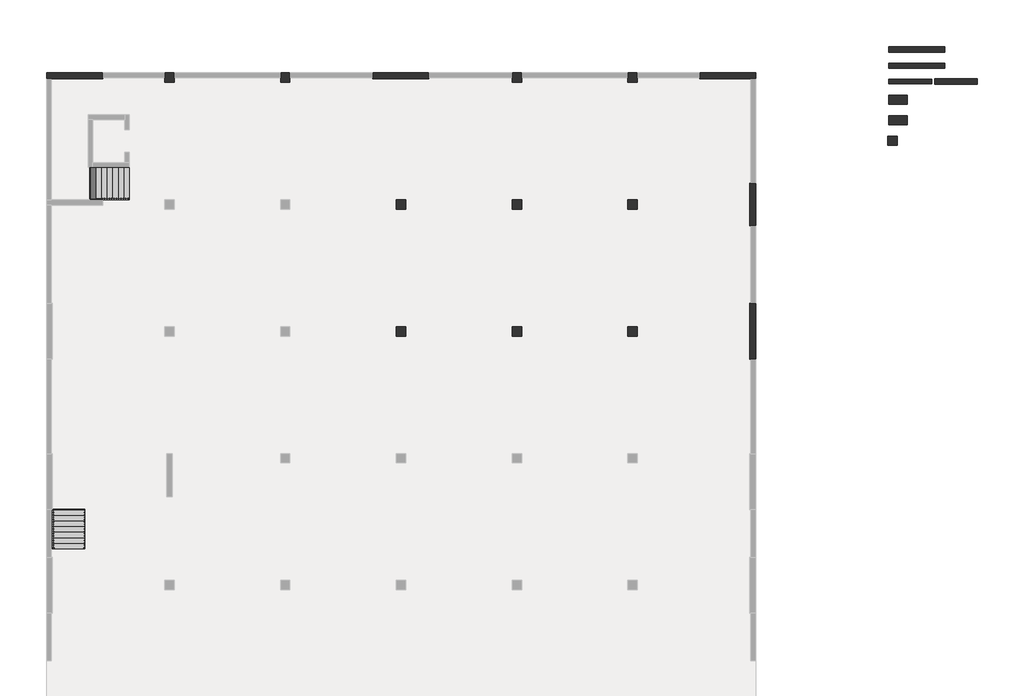
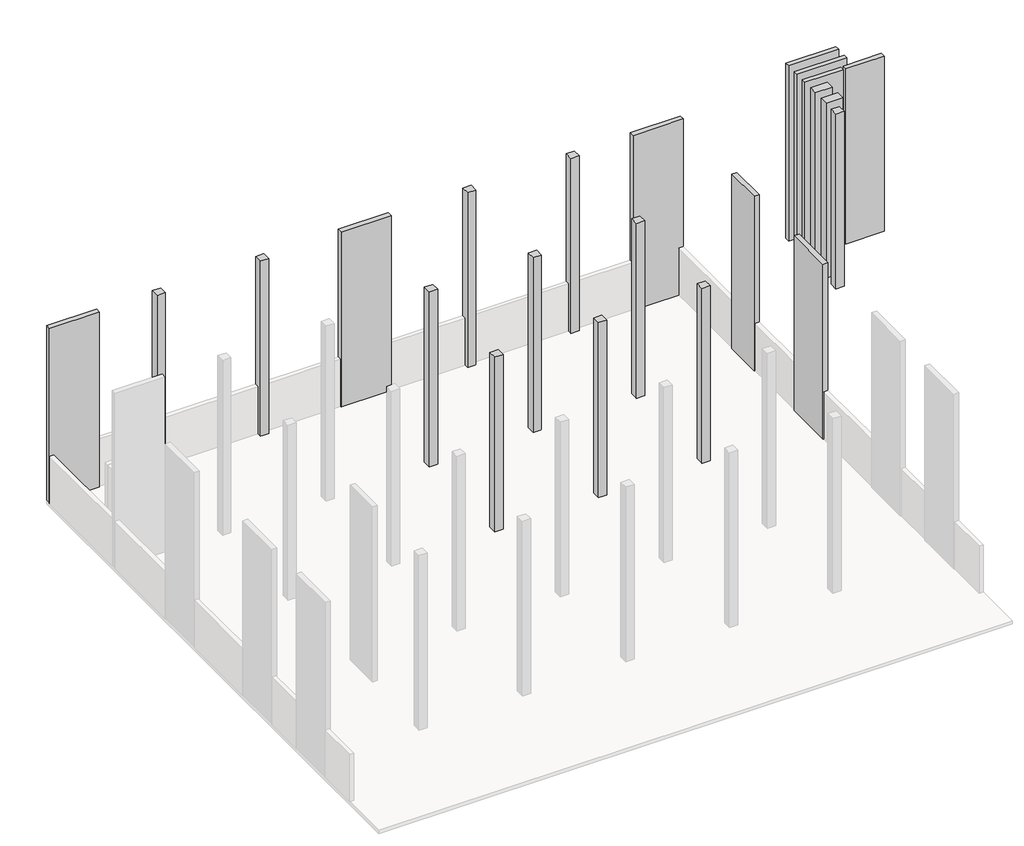
# One storey, part 2 of 2: 22 columns, 3 railings, 2 members, 2 stair flights.
"""IFC4 building model written with IfcOpenShell, lengths in millimetres."""

import ifcopenshell
import ifcopenshell.guid

model = None  # the IFC model being written
_history = None  # IfcOwnerHistory: only IFC2X3 demands one
_inside = {}  # id of a spatial element -> (the spatial element, [elements in it])
_under = {}  # id of a project, library or spatial element -> (it, [spatial elements below it])
_declared = {}  # id of a project -> (the project, [libraries it declares])
_typed = {}  # id of a type object -> (the type object, [elements of that type])
_made_of = {}  # id of a material, layer set ... -> (it, [elements and type objects made of it])


def new_model(schema):
    """Start an empty IFC model of exactly this schema.

    Asked for "IFC4X3", IfcOpenShell would pick the latest addendum, in which some entities
    have other attributes; the version numbers below select the first issue.
    IFC2X3 requires an IfcOwnerHistory on every rooted entity: one is made here for all.
    """
    global model, _history
    if schema == "IFC4X3":
        model = ifcopenshell.file(schema_version=(4, 3, 0, 0))
    else:
        model = ifcopenshell.file(schema=schema)
    _inside.clear()
    _under.clear()
    _declared.clear()
    _typed.clear()
    _made_of.clear()
    _history = None
    if model.schema == "IFC2X3":
        org = make("IfcOrganization", Name="unknown")
        user = make(
            "IfcPersonAndOrganization",
            ThePerson=make("IfcPerson", FamilyName="unknown"),
            TheOrganization=org,
        )
        app = make(
            "IfcApplication",
            ApplicationDeveloper=org,
            Version="unknown",
            ApplicationFullName="unknown",
            ApplicationIdentifier="unknown",
        )
        _history = make(
            "IfcOwnerHistory",
            OwningUser=user,
            OwningApplication=app,
            ChangeAction="ADDED",
            CreationDate=0,
        )
    return model


def make(cls, **values):
    """One entity of the class cls with the attributes given. An attribute that is None is left unset."""
    return model.create_entity(
        cls, **{name: value for name, value in values.items() if value is not None}
    )


def rooted(cls, **values):
    """An entity with a GlobalId (a new one), such as an element, a storey or a relation."""
    return make(cls, GlobalId=ifcopenshell.guid.new(), OwnerHistory=_history, **values)


def si_unit(unit_type, name, prefix=None):
    """IfcSIUnit, for example si_unit("LENGTHUNIT", "METRE", prefix="MILLI")."""
    return make("IfcSIUnit", UnitType=unit_type, Prefix=prefix, Name=name)


def assignment(units):
    """IfcUnitAssignment: the units of a project."""
    return None if units is None else make("IfcUnitAssignment", Units=units)


def point(xyz):
    """IfcCartesianPoint."""
    return None if xyz is None else make("IfcCartesianPoint", Coordinates=xyz)


def direction(xyz):
    """IfcDirection."""
    return None if xyz is None else make("IfcDirection", DirectionRatios=xyz)


def frame(location, z_axis=None, x_axis=None):
    """IfcAxis2Placement3D, a coordinate frame: its origin and axes. An axis left out is left unset."""
    return make(
        "IfcAxis2Placement3D",
        Location=point(location),
        Axis=direction(z_axis),
        RefDirection=direction(x_axis),
    )


def origin():
    """The frame at (0, 0, 0) with its axes left unset."""
    return frame((0.0, 0.0, 0.0))


def place(relative_to, where):
    """IfcLocalPlacement: puts the frame where relative to a parent placement (None: the world)."""
    return make(
        "IfcLocalPlacement", PlacementRelTo=relative_to, RelativePlacement=where
    )


def context(
    kind, dimensions, precision=None, world=None, true_north=None, identifier=None
):
    """IfcGeometricRepresentationContext, for example the 3D "Model" context."""
    return make(
        "IfcGeometricRepresentationContext",
        ContextIdentifier=identifier,
        ContextType=kind,
        CoordinateSpaceDimension=dimensions,
        Precision=precision,
        WorldCoordinateSystem=world,
        TrueNorth=true_north,
    )


def project(units=None, contexts=None):
    """IfcProject with its units and contexts."""
    return rooted(
        "IfcProject",
        Name="project",
        RepresentationContexts=contexts,
        UnitsInContext=assignment(units),
    )


def spatial(cls, under=None, at=None, **own):
    """A site, building, storey or space (cls), placed at a placement, below another one or the project."""
    s = rooted(cls, ObjectPlacement=at, **own)
    if under is not None:
        _under.setdefault(under.id(), (under, []))[1].append(s)
    return s


def polyline(points):
    """IfcPolyline through the points."""
    return make("IfcPolyline", Points=[point(p) for p in points])


def outline(outer, holes=None, kind="AREA"):
    """IfcArbitraryClosedProfileDef: a profile drawn as a closed curve; with holes, ...WithVoids."""
    if holes is None:
        return make("IfcArbitraryClosedProfileDef", ProfileType=kind, OuterCurve=outer)
    return make(
        "IfcArbitraryProfileDefWithVoids",
        ProfileType=kind,
        OuterCurve=outer,
        InnerCurves=holes,
    )


def extrude(swept, where, along, depth):
    """IfcExtrudedAreaSolid: the profile swept, set in the frame where, extruded along a direction by depth."""
    return make(
        "IfcExtrudedAreaSolid",
        SweptArea=swept,
        Position=where,
        ExtrudedDirection=direction(along),
        Depth=depth,
    )


def shape(context_of_items, identifier, shape_type, items):
    """IfcShapeRepresentation: the items that make up one representation, for example the "Body"."""
    return make(
        "IfcShapeRepresentation",
        ContextOfItems=context_of_items,
        RepresentationIdentifier=identifier,
        RepresentationType=shape_type,
        Items=items,
    )


def source(mapping_origin, context_of_items, identifier, shape_type, items):
    """IfcRepresentationMap: a shape defined once, which mapped items show again and again."""
    return make(
        "IfcRepresentationMap",
        MappingOrigin=mapping_origin,
        MappedRepresentation=shape(context_of_items, identifier, shape_type, items),
    )


def transform(
    local_origin,
    x_axis=None,
    y_axis=None,
    z_axis=None,
    scale=None,
    scale2=None,
    scale3=None,
    uniform=True,
):
    """IfcCartesianTransformationOperator3D, or its non-uniform kind. x_axis, y_axis, z_axis: its Axis1, 2, 3."""
    if uniform:
        return make(
            "IfcCartesianTransformationOperator3D",
            Axis1=direction(x_axis),
            Axis2=direction(y_axis),
            LocalOrigin=point(local_origin),
            Scale=scale,
            Axis3=direction(z_axis),
        )
    return make(
        "IfcCartesianTransformationOperator3DnonUniform",
        Axis1=direction(x_axis),
        Axis2=direction(y_axis),
        LocalOrigin=point(local_origin),
        Scale=scale,
        Axis3=direction(z_axis),
        Scale2=scale2,
        Scale3=scale3,
    )


def mapped(mapping_source, mapping_target):
    """IfcMappedItem: shows the shape of a source again, moved by a transform."""
    return make(
        "IfcMappedItem", MappingSource=mapping_source, MappingTarget=mapping_target
    )


def made_of(thing, what):
    """Note that an element or type object is made of a material, layer set ...; save() writes the relation."""
    if what is not None:
        _made_of.setdefault(what.id(), (what, []))[1].append(thing)
    return thing


def element(
    cls,
    number,
    at=None,
    inside=None,
    cuts=None,
    type_object=None,
    material=None,
    context=None,
    identifier="Body",
    shape_type=None,
    held_by="IfcProductDefinitionShape",
    body=None,
    shapes=None,
    **own,
):
    """One element of the class cls, such as IfcWall. Its Tag is "e" and its number.

    at: its placement. inside: the storey or other place that contains it. cuts: it is an
    opening in that element (IfcRelVoidsElement). A single representation is given by context,
    identifier, shape_type and body (its items); several are given by shapes. held_by: the class
    of the entity that holds the representations. save() writes the other relations.
    """
    e = rooted(cls, Tag="e%d" % number, ObjectPlacement=at, **own)
    if body is not None:
        shapes = [shape(context, identifier, shape_type, body)]
    if shapes is not None:
        e.Representation = make(held_by, Representations=shapes)
    if inside is not None:
        _inside.setdefault(inside.id(), (inside, []))[1].append(e)
    if cuts is not None:
        rooted(
            "IfcRelVoidsElement", RelatingBuildingElement=cuts, RelatedOpeningElement=e
        )
    if type_object is not None:
        _typed.setdefault(type_object.id(), (type_object, []))[1].append(e)
    return made_of(e, material)


def aggregate(whole, parts):
    """IfcRelAggregates: a whole, such as a stair, and the parts it consists of."""
    return rooted("IfcRelAggregates", RelatingObject=whole, RelatedObjects=parts)


def save(model, path):
    """Write the relations noted so far, then the file.

    IfcRelAggregates (storeys below a building ...), IfcRelContainedInSpatialStructure (elements
    in a storey), IfcRelDefinesByType, IfcRelAssociatesMaterial and IfcRelDeclares: one each for
    every whole, place, type object, material and project.
    """
    for whole, parts in _under.values():
        aggregate(whole, parts)
    for where, things in _inside.values():
        rooted(
            "IfcRelContainedInSpatialStructure",
            RelatedElements=things,
            RelatingStructure=where,
        )
    for kind, things in _typed.values():
        rooted("IfcRelDefinesByType", RelatedObjects=things, RelatingType=kind)
    for what, things in _made_of.values():
        rooted("IfcRelAssociatesMaterial", RelatedObjects=things, RelatingMaterial=what)
    for by, libraries in _declared.values():
        rooted("IfcRelDeclares", RelatingContext=by, RelatedDefinitions=libraries)
    model.write(path)


def m_rectangular_column_100x50_89a3459c(model_context):
    return source(origin(), model_context, "Body", "SweptSolid", [
        extrude(outline(polyline([(500.0, 250.0), (500.0, -250.0), (-500.0, -250.0), (-500.0, 250.0), (500.0, 250.0)])), frame((0.0, 0.0, -3200.0), z_axis=(0.0, 0.0, 1.0), x_axis=(1.0, 0.0, 0.0)), (0.0, 0.0, 1.0), 11100.0),
    ])


def m_rectangular_column_230x25_da6e8c6c(model_context):
    return source(origin(), model_context, "Body", "SweptSolid", [
        extrude(outline(polyline([(1150.0, 125.0), (1150.0, -125.0), (-1150.0, -125.0), (-1150.0, 125.0), (1150.0, 125.0)])), frame((0.0, 0.0, -3200.0), z_axis=(0.0, 0.0, 1.0), x_axis=(1.0, 0.0, 0.0)), (0.0, 0.0, 1.0), 11100.0),
    ])


def m_rectangular_column_230x30_624f9335(model_context):
    return source(origin(), model_context, "Body", "SweptSolid", [
        extrude(outline(polyline([(1150.0, 150.0), (1150.0, -150.0), (-1150.0, -150.0), (-1150.0, 150.0), (1150.0, 150.0)])), frame((0.0, 0.0, -3200.0), z_axis=(0.0, 0.0, 1.0), x_axis=(1.0, 0.0, 0.0)), (0.0, 0.0, 1.0), 11100.0),
    ])


def m_rectangular_column_300x25_b7e4e278(model_context):
    return source(origin(), model_context, "Body", "SweptSolid", [
        extrude(outline(polyline([(1500.0, 125.0), (1500.0, -125.0), (-1500.0, -125.0), (-1500.0, 125.0), (1500.0, 125.0)])), frame((0.0, 0.0, -3200.0), z_axis=(0.0, 0.0, 1.0), x_axis=(1.0, 0.0, 0.0)), (0.0, 0.0, 1.0), 11100.0),
    ])


def m_rectangular_column_300x30_b7aa0491(model_context):
    return source(origin(), model_context, "Body", "SweptSolid", [
        extrude(outline(polyline([(1500.0, 150.0), (1500.0, -150.0), (-1500.0, -150.0), (-1500.0, 150.0), (1500.0, 150.0)])), frame((0.0, 0.0, -3200.0), z_axis=(0.0, 0.0, 1.0), x_axis=(1.0, 0.0, 0.0)), (0.0, 0.0, 1.0), 11100.0),
    ])


def m_rectangular_column_50x50_3a95f3c9(model_context):
    return source(origin(), model_context, "Body", "SweptSolid", [
        extrude(outline(polyline([(250.0, 250.0), (250.0, -250.0), (-250.0, -250.0), (-250.0, 250.0), (250.0, 250.0)])), frame((0.0, 0.0, -3200.0), z_axis=(0.0, 0.0, 1.0), x_axis=(1.0, 0.0, 0.0)), (0.0, 0.0, 1.0), 11100.0),
    ])


def stair_flight_50mm_tread_13mm_riser_a4aa0c66(model_context):
    return source(origin(), model_context, "Body", "SweptSolid", [
        extrude(outline(polyline([(-13456.918089, 12730.6768963), (-13444.418089, 12730.6768963), (-13444.418089, 11030.6768963), (-13456.918089, 11030.6768963), (-13456.918089, 12730.6768963)])), frame((0.0, 0.0, -3200.0), z_axis=(0.0, 0.0, 1.0), x_axis=(1.0, 0.0, 0.0)), (0.0, 0.0, 1.0), 127.7777778),
        extrude(outline(polyline([(-13744.418089, 11030.6768963), (-13744.418089, 12730.6768963), (-13444.418089, 12730.6768963), (-13444.418089, 11030.6768963), (-13744.418089, 11030.6768963)])), frame((0.0, 0.0, -3072.2222222), z_axis=(0.0, 0.0, 1.0), x_axis=(1.0, 0.0, 0.0)), (0.0, 0.0, 1.0), 50.0),
        extrude(outline(polyline([(-13756.918089, 12730.6768963), (-13744.418089, 12730.6768963), (-13744.418089, 11030.6768963), (-13756.918089, 11030.6768963), (-13756.918089, 12730.6768963)])), frame((0.0, 0.0, -3072.2222222), z_axis=(0.0, 0.0, 1.0), x_axis=(1.0, 0.0, 0.0)), (0.0, 0.0, 1.0), 177.7777778),
        extrude(outline(polyline([(-14044.418089, 11030.6768963), (-14044.418089, 12730.6768963), (-13744.418089, 12730.6768963), (-13744.418089, 11030.6768963), (-14044.418089, 11030.6768963)])), frame((0.0, 0.0, -2894.4444444), z_axis=(0.0, 0.0, 1.0), x_axis=(1.0, 0.0, 0.0)), (0.0, 0.0, 1.0), 50.0),
        extrude(outline(polyline([(-14056.918089, 12730.6768963), (-14044.418089, 12730.6768963), (-14044.418089, 11030.6768963), (-14056.918089, 11030.6768963), (-14056.918089, 12730.6768963)])), frame((0.0, 0.0, -2894.4444444), z_axis=(0.0, 0.0, 1.0), x_axis=(1.0, 0.0, 0.0)), (0.0, 0.0, 1.0), 177.7777778),
        extrude(outline(polyline([(-14344.418089, 11030.6768963), (-14344.418089, 12730.6768963), (-14044.418089, 12730.6768963), (-14044.418089, 11030.6768963), (-14344.418089, 11030.6768963)])), frame((0.0, 0.0, -2716.6666667), z_axis=(0.0, 0.0, 1.0), x_axis=(1.0, 0.0, 0.0)), (0.0, 0.0, 1.0), 50.0),
        extrude(outline(polyline([(-14356.918089, 12730.6768963), (-14344.418089, 12730.6768963), (-14344.418089, 11030.6768963), (-14356.918089, 11030.6768963), (-14356.918089, 12730.6768963)])), frame((0.0, 0.0, -2716.6666667), z_axis=(0.0, 0.0, 1.0), x_axis=(1.0, 0.0, 0.0)), (0.0, 0.0, 1.0), 177.7777778),
        extrude(outline(polyline([(-14644.418089, 11030.6768963), (-14644.418089, 12730.6768963), (-14344.418089, 12730.6768963), (-14344.418089, 11030.6768963), (-14644.418089, 11030.6768963)])), frame((0.0, 0.0, -2538.8888889), z_axis=(0.0, 0.0, 1.0), x_axis=(1.0, 0.0, 0.0)), (0.0, 0.0, 1.0), 50.0),
        extrude(outline(polyline([(-14656.918089, 12730.6768963), (-14644.418089, 12730.6768963), (-14644.418089, 11030.6768963), (-14656.918089, 11030.6768963), (-14656.918089, 12730.6768963)])), frame((0.0, 0.0, -2538.8888889), z_axis=(0.0, 0.0, 1.0), x_axis=(1.0, 0.0, 0.0)), (0.0, 0.0, 1.0), 177.7777778),
        extrude(outline(polyline([(-14944.418089, 11030.6768963), (-14944.418089, 12730.6768963), (-14644.418089, 12730.6768963), (-14644.418089, 11030.6768963), (-14944.418089, 11030.6768963)])), frame((0.0, 0.0, -2361.1111111), z_axis=(0.0, 0.0, 1.0), x_axis=(1.0, 0.0, 0.0)), (0.0, 0.0, 1.0), 50.0),
        extrude(outline(polyline([(-14956.918089, 12730.6768963), (-14944.418089, 12730.6768963), (-14944.418089, 11030.6768963), (-14956.918089, 11030.6768963), (-14956.918089, 12730.6768963)])), frame((0.0, 0.0, -2361.1111111), z_axis=(0.0, 0.0, 1.0), x_axis=(1.0, 0.0, 0.0)), (0.0, 0.0, 1.0), 177.7777778),
        extrude(outline(polyline([(-15244.418089, 11030.6768963), (-15244.418089, 12730.6768963), (-14944.418089, 12730.6768963), (-14944.418089, 11030.6768963), (-15244.418089, 11030.6768963)])), frame((0.0, 0.0, -2183.3333333), z_axis=(0.0, 0.0, 1.0), x_axis=(1.0, 0.0, 0.0)), (0.0, 0.0, 1.0), 50.0),
        extrude(outline(polyline([(-15256.918089, 12730.6768963), (-15244.418089, 12730.6768963), (-15244.418089, 11030.6768963), (-15256.918089, 11030.6768963), (-15256.918089, 12730.6768963)])), frame((0.0, 0.0, -2183.3333333), z_axis=(0.0, 0.0, 1.0), x_axis=(1.0, 0.0, 0.0)), (0.0, 0.0, 1.0), 177.7777778),
        extrude(outline(polyline([(-15556.918089, 12730.6768963), (-15544.418089, 12730.6768963), (-15544.418089, 11030.6768963), (-15556.918089, 11030.6768963), (-15556.918089, 12730.6768963)])), frame((0.0, 0.0, -2005.5555556), z_axis=(0.0, 0.0, 1.0), x_axis=(1.0, 0.0, 0.0)), (0.0, 0.0, 1.0), 177.7777778),
        extrude(outline(polyline([(-15544.418089, 11030.6768963), (-15544.418089, 12730.6768963), (-15244.418089, 12730.6768963), (-15244.418089, 11030.6768963), (-15544.418089, 11030.6768963)])), frame((0.0, 0.0, -2005.5555556), z_axis=(0.0, 0.0, 1.0), x_axis=(1.0, 0.0, 0.0)), (0.0, 0.0, 1.0), 50.0),
    ])


def stair_flight_50mm_tread_13mm_riser_6111fc84(model_context):
    return source(origin(), model_context, "Body", "SweptSolid", [
        extrude(outline(polyline([(-15825.2814495, -7705.5731037), (-15825.2814495, -7718.0731037), (-17525.2814495, -7718.0731037), (-17525.2814495, -7705.5731037), (-15825.2814495, -7705.5731037)])), frame((0.0, 0.0, -3200.0), z_axis=(0.0, 0.0, 1.0), x_axis=(1.0, 0.0, 0.0)), (0.0, 0.0, 1.0), 83.3333333),
        extrude(outline(polyline([(-17525.2814495, -7418.0731037), (-15825.2814495, -7418.0731037), (-15825.2814495, -7718.0731037), (-17525.2814495, -7718.0731037), (-17525.2814495, -7418.0731037)])), frame((0.0, 0.0, -3116.6666667), z_axis=(0.0, 0.0, 1.0), x_axis=(1.0, 0.0, 0.0)), (0.0, 0.0, 1.0), 50.0),
        extrude(outline(polyline([(-15825.2814495, -7405.5731037), (-15825.2814495, -7418.0731037), (-17525.2814495, -7418.0731037), (-17525.2814495, -7405.5731037), (-15825.2814495, -7405.5731037)])), frame((0.0, 0.0, -3116.6666667), z_axis=(0.0, 0.0, 1.0), x_axis=(1.0, 0.0, 0.0)), (0.0, 0.0, 1.0), 133.3333333),
        extrude(outline(polyline([(-17525.2814495, -7118.0731037), (-15825.2814495, -7118.0731037), (-15825.2814495, -7418.0731037), (-17525.2814495, -7418.0731037), (-17525.2814495, -7118.0731037)])), frame((0.0, 0.0, -2983.3333333), z_axis=(0.0, 0.0, 1.0), x_axis=(1.0, 0.0, 0.0)), (0.0, 0.0, 1.0), 50.0),
        extrude(outline(polyline([(-15825.2814495, -7105.5731037), (-15825.2814495, -7118.0731037), (-17525.2814495, -7118.0731037), (-17525.2814495, -7105.5731037), (-15825.2814495, -7105.5731037)])), frame((0.0, 0.0, -2983.3333333), z_axis=(0.0, 0.0, 1.0), x_axis=(1.0, 0.0, 0.0)), (0.0, 0.0, 1.0), 133.3333333),
        extrude(outline(polyline([(-17525.2814495, -6818.0731037), (-15825.2814495, -6818.0731037), (-15825.2814495, -7118.0731037), (-17525.2814495, -7118.0731037), (-17525.2814495, -6818.0731037)])), frame((0.0, 0.0, -2850.0), z_axis=(0.0, 0.0, 1.0), x_axis=(1.0, 0.0, 0.0)), (0.0, 0.0, 1.0), 50.0),
        extrude(outline(polyline([(-15825.2814495, -6805.5731037), (-15825.2814495, -6818.0731037), (-17525.2814495, -6818.0731037), (-17525.2814495, -6805.5731037), (-15825.2814495, -6805.5731037)])), frame((0.0, 0.0, -2850.0), z_axis=(0.0, 0.0, 1.0), x_axis=(1.0, 0.0, 0.0)), (0.0, 0.0, 1.0), 133.3333333),
        extrude(outline(polyline([(-17525.2814495, -6518.0731037), (-15825.2814495, -6518.0731037), (-15825.2814495, -6818.0731037), (-17525.2814495, -6818.0731037), (-17525.2814495, -6518.0731037)])), frame((0.0, 0.0, -2716.6666667), z_axis=(0.0, 0.0, 1.0), x_axis=(1.0, 0.0, 0.0)), (0.0, 0.0, 1.0), 50.0),
        extrude(outline(polyline([(-15825.2814495, -6505.5731037), (-15825.2814495, -6518.0731037), (-17525.2814495, -6518.0731037), (-17525.2814495, -6505.5731037), (-15825.2814495, -6505.5731037)])), frame((0.0, 0.0, -2716.6666667), z_axis=(0.0, 0.0, 1.0), x_axis=(1.0, 0.0, 0.0)), (0.0, 0.0, 1.0), 133.3333333),
        extrude(outline(polyline([(-17525.2814495, -6218.0731037), (-15825.2814495, -6218.0731037), (-15825.2814495, -6518.0731037), (-17525.2814495, -6518.0731037), (-17525.2814495, -6218.0731037)])), frame((0.0, 0.0, -2583.3333333), z_axis=(0.0, 0.0, 1.0), x_axis=(1.0, 0.0, 0.0)), (0.0, 0.0, 1.0), 50.0),
        extrude(outline(polyline([(-15825.2814495, -6205.5731037), (-15825.2814495, -6218.0731037), (-17525.2814495, -6218.0731037), (-17525.2814495, -6205.5731037), (-15825.2814495, -6205.5731037)])), frame((0.0, 0.0, -2583.3333333), z_axis=(0.0, 0.0, 1.0), x_axis=(1.0, 0.0, 0.0)), (0.0, 0.0, 1.0), 133.3333333),
        extrude(outline(polyline([(-17525.2814495, -5918.0731037), (-15825.2814495, -5918.0731037), (-15825.2814495, -6218.0731037), (-17525.2814495, -6218.0731037), (-17525.2814495, -5918.0731037)])), frame((0.0, 0.0, -2450.0), z_axis=(0.0, 0.0, 1.0), x_axis=(1.0, 0.0, 0.0)), (0.0, 0.0, 1.0), 50.0),
        extrude(outline(polyline([(-15825.2814495, -5905.5731037), (-15825.2814495, -5918.0731037), (-17525.2814495, -5918.0731037), (-17525.2814495, -5905.5731037), (-15825.2814495, -5905.5731037)])), frame((0.0, 0.0, -2450.0), z_axis=(0.0, 0.0, 1.0), x_axis=(1.0, 0.0, 0.0)), (0.0, 0.0, 1.0), 133.3333333),
        extrude(outline(polyline([(-15825.2814495, -5605.5731037), (-15825.2814495, -5618.0731037), (-17525.2814495, -5618.0731037), (-17525.2814495, -5605.5731037), (-15825.2814495, -5605.5731037)])), frame((0.0, 0.0, -2316.6666667), z_axis=(0.0, 0.0, 1.0), x_axis=(1.0, 0.0, 0.0)), (0.0, 0.0, 1.0), 133.3333333),
        extrude(outline(polyline([(-17525.2814495, -5618.0731037), (-15825.2814495, -5618.0731037), (-15825.2814495, -5918.0731037), (-17525.2814495, -5918.0731037), (-17525.2814495, -5618.0731037)])), frame((0.0, 0.0, -2316.6666667), z_axis=(0.0, 0.0, 1.0), x_axis=(1.0, 0.0, 0.0)), (0.0, 0.0, 1.0), 50.0),
    ])


model = new_model("IFC4")

# Units and contexts
model_context = context("Model", 3, world=origin())
ifc_project = project(units=[si_unit("LENGTHUNIT", "METRE", prefix="MILLI")], contexts=[model_context])

# Site, building, storey
site = spatial("IfcSite", under=ifc_project)
building = spatial("IfcBuilding", under=site)
storey = spatial("IfcBuildingStorey", under=building, Name="Bodrumi", Elevation=-3200.0)

# Columns
placement = place(None, origin())
m_rectangular_column_100x50_shape = m_rectangular_column_100x50_89a3459c(model_context)
element("IfcColumn", 1, ObjectType="M_Rectangular Column : 100x50", at=placement, inside=storey, context=model_context, shape_type="MappedRepresentation", body=[
    mapped(m_rectangular_column_100x50_shape, transform((27767.4045961, 16346.6713325, 0.0), x_axis=(1.0, 0.0, 0.0), y_axis=(0.0, 1.0, 0.0), z_axis=(0.0, 0.0, 1.0))),
])
element("IfcColumn", 2, ObjectType="M_Rectangular Column : 100x50", at=placement, inside=storey, context=model_context, shape_type="MappedRepresentation", body=[
    mapped(m_rectangular_column_100x50_shape, transform((27767.4045961, 15246.6713325, 0.0), x_axis=(1.0, 0.0, 0.0), y_axis=(0.0, 1.0, 0.0), z_axis=(0.0, 0.0, 1.0))),
])
m_rectangular_column_230x25_shape = m_rectangular_column_230x25_da6e8c6c(model_context)
element("IfcColumn", 3, ObjectType="M_Rectangular Column : 230x25", at=placement, inside=storey, context=model_context, shape_type="MappedRepresentation", body=[
    mapped(m_rectangular_column_230x25_shape, transform((28417.4045961, 17321.6713325, 0.0), x_axis=(1.0, 0.0, 0.0), y_axis=(0.0, 1.0, 0.0), z_axis=(0.0, 0.0, 1.0))),
])
m_rectangular_column_230x30_shape = m_rectangular_column_230x30_624f9335(model_context)
element("IfcColumn", 4, ObjectType="M_Rectangular Column : 230x30", at=placement, inside=storey, context=model_context, shape_type="MappedRepresentation", body=[
    mapped(m_rectangular_column_230x30_shape, transform((30867.9046685, 17321.6713325, 0.0), x_axis=(1.0, 0.0, 0.0), y_axis=(0.0, 1.0, 0.0), z_axis=(0.0, 0.0, 1.0))),
])
element("IfcColumn", 5, ObjectType="M_Rectangular Column : 230x30", at=placement, inside=storey, context=model_context, shape_type="MappedRepresentation", body=[
    mapped(m_rectangular_column_230x30_shape, transform((19975.581911, 10730.6768963, 0.0), x_axis=(0.0, 1.0, 0.0), y_axis=(-1.0, 0.0, 0.0), z_axis=(0.0, 0.0, 1.0))),
])
m_rectangular_column_300x25_shape = m_rectangular_column_300x25_b7e4e278(model_context)
element("IfcColumn", 6, ObjectType="M_Rectangular Column : 300x25", at=placement, inside=storey, context=model_context, shape_type="MappedRepresentation", body=[
    mapped(m_rectangular_column_300x25_shape, transform((28767.4045961, 18171.6713325, 0.0), x_axis=(1.0, 0.0, 0.0), y_axis=(0.0, 1.0, 0.0), z_axis=(0.0, 0.0, 1.0))),
])
element("IfcColumn", 7, ObjectType="M_Rectangular Column : 300x30", at=placement, inside=storey, context=model_context, shape_type="SweptSolid", body=[
    extrude(outline(polyline([(-14874.418089, 17780.6768963), (-14874.418089, 17480.6768963), (-17874.418089, 17480.6768963), (-17874.418089, 17780.6768963), (-14874.418089, 17780.6768963)])), frame((0.0, 0.0, -3200.0), z_axis=(0.0, 0.0, 1.0), x_axis=(1.0, 0.0, 0.0)), (0.0, 0.0, 1.0), 11100.0),
])
m_rectangular_column_300x30_shape = m_rectangular_column_300x30_b7aa0491(model_context)
element("IfcColumn", 8, ObjectType="M_Rectangular Column : 300x30", at=placement, inside=storey, context=model_context, shape_type="MappedRepresentation", body=[
    mapped(m_rectangular_column_300x30_shape, transform((28767.4045961, 19046.6713325, 0.0), x_axis=(1.0, 0.0, 0.0), y_axis=(0.0, 1.0, 0.0), z_axis=(0.0, 0.0, 1.0))),
])
element("IfcColumn", 9, ObjectType="M_Rectangular Column : 300x30", at=placement, inside=storey, context=model_context, shape_type="MappedRepresentation", body=[
    mapped(m_rectangular_column_300x30_shape, transform((18625.581911, 17630.6768963, 0.0), x_axis=(1.0, 0.0, 0.0), y_axis=(0.0, 1.0, 0.0), z_axis=(0.0, 0.0, 1.0))),
])
element("IfcColumn", 10, ObjectType="M_Rectangular Column : 300x30", at=placement, inside=storey, context=model_context, shape_type="MappedRepresentation", body=[
    mapped(m_rectangular_column_300x30_shape, transform((1115.581911, 17630.6768963, 0.0), x_axis=(1.0, 0.0, 0.0), y_axis=(0.0, 1.0, 0.0), z_axis=(0.0, 0.0, 1.0))),
])
element("IfcColumn", 11, ObjectType="M_Rectangular Column : 300x30", at=placement, inside=storey, context=model_context, shape_type="MappedRepresentation", body=[
    mapped(m_rectangular_column_300x30_shape, transform((19975.581911, 3930.6768963, 0.0), x_axis=(0.0, 1.0, 0.0), y_axis=(-1.0, 0.0, 0.0), z_axis=(0.0, 0.0, 1.0))),
])
m_rectangular_column_50x50_shape = m_rectangular_column_50x50_3a95f3c9(model_context)
element("IfcColumn", 12, ObjectType="M_Rectangular Column : 50x50", at=placement, inside=storey, context=model_context, shape_type="MappedRepresentation", body=[
    mapped(m_rectangular_column_50x50_shape, transform((27471.1352536, 14146.6713325, 0.0), x_axis=(1.0, 0.0, 0.0), y_axis=(0.0, 1.0, 0.0), z_axis=(0.0, 0.0, 1.0))),
])
element("IfcColumn", 13, ObjectType="M_Rectangular Column : 50x50", at=placement, inside=storey, context=model_context, shape_type="MappedRepresentation", body=[
    mapped(m_rectangular_column_50x50_shape, transform((13535.581911, 3930.6768963, 0.0), x_axis=(1.0, 0.0, 0.0), y_axis=(0.0, 1.0, 0.0), z_axis=(0.0, 0.0, 1.0))),
])
element("IfcColumn", 14, ObjectType="M_Rectangular Column : 50x50", at=placement, inside=storey, context=model_context, shape_type="MappedRepresentation", body=[
    mapped(m_rectangular_column_50x50_shape, transform((13535.581911, 17530.6768963, 0.0), x_axis=(1.0, 0.0, 0.0), y_axis=(0.0, 1.0, 0.0), z_axis=(0.0, 0.0, 1.0))),
])
element("IfcColumn", 15, ObjectType="M_Rectangular Column : 50x50", at=placement, inside=storey, context=model_context, shape_type="MappedRepresentation", body=[
    mapped(m_rectangular_column_50x50_shape, transform((7335.581911, 17530.6768963, 0.0), x_axis=(1.0, 0.0, 0.0), y_axis=(0.0, 1.0, 0.0), z_axis=(0.0, 0.0, 1.0))),
])
element("IfcColumn", 16, ObjectType="M_Rectangular Column : 50x50", at=placement, inside=storey, context=model_context, shape_type="MappedRepresentation", body=[
    mapped(m_rectangular_column_50x50_shape, transform((-5084.418089, 17530.6768963, 0.0), x_axis=(1.0, 0.0, 0.0), y_axis=(0.0, 1.0, 0.0), z_axis=(0.0, 0.0, 1.0))),
])
element("IfcColumn", 17, ObjectType="M_Rectangular Column : 50x50", at=placement, inside=storey, context=model_context, shape_type="MappedRepresentation", body=[
    mapped(m_rectangular_column_50x50_shape, transform((-11284.418089, 17530.6768963, 0.0), x_axis=(1.0, 0.0, 0.0), y_axis=(0.0, 1.0, 0.0), z_axis=(0.0, 0.0, 1.0))),
])
element("IfcColumn", 18, ObjectType="M_Rectangular Column : 50x50", at=placement, inside=storey, context=model_context, shape_type="MappedRepresentation", body=[
    mapped(m_rectangular_column_50x50_shape, transform((1115.581911, 10730.6768963, 0.0), x_axis=(1.0, 0.0, 0.0), y_axis=(0.0, 1.0, 0.0), z_axis=(0.0, 0.0, 1.0))),
])
element("IfcColumn", 19, ObjectType="M_Rectangular Column : 50x50", at=placement, inside=storey, context=model_context, shape_type="MappedRepresentation", body=[
    mapped(m_rectangular_column_50x50_shape, transform((7335.581911, 10730.6768963, 0.0), x_axis=(1.0, 0.0, 0.0), y_axis=(0.0, 1.0, 0.0), z_axis=(0.0, 0.0, 1.0))),
])
element("IfcColumn", 20, ObjectType="M_Rectangular Column : 50x50", at=placement, inside=storey, context=model_context, shape_type="MappedRepresentation", body=[
    mapped(m_rectangular_column_50x50_shape, transform((13535.581911, 10730.6768963, 0.0), x_axis=(1.0, 0.0, 0.0), y_axis=(0.0, 1.0, 0.0), z_axis=(0.0, 0.0, 1.0))),
])
element("IfcColumn", 21, ObjectType="M_Rectangular Column : 50x50", at=placement, inside=storey, context=model_context, shape_type="MappedRepresentation", body=[
    mapped(m_rectangular_column_50x50_shape, transform((1115.581911, 3930.6768963, 0.0), x_axis=(1.0, 0.0, 0.0), y_axis=(0.0, 1.0, 0.0), z_axis=(0.0, 0.0, 1.0))),
])
element("IfcColumn", 22, ObjectType="M_Rectangular Column : 50x50", at=placement, inside=storey, context=model_context, shape_type="MappedRepresentation", body=[
    mapped(m_rectangular_column_50x50_shape, transform((7335.581911, 3930.6768963, 0.0), x_axis=(1.0, 0.0, 0.0), y_axis=(0.0, 1.0, 0.0), z_axis=(0.0, 0.0, 1.0))),
])

# Members
element("IfcMember", 23, ObjectType="Stringer - 50mm Width", at=placement, inside=storey, context=model_context, shape_type="SweptSolid", body=[
    extrude(outline(polyline([(-3200.0, -13444.418089), (-2966.808244, -13444.418089), (-1722.3637995, -15544.418089), (-2187.322461, -15544.418089), (-3200.0, -13835.524742), (-3200.0, -13444.418089)])), frame((0.0, 10980.6768963, 0.0), z_axis=(0.0, 1.0, 0.0), x_axis=(0.0, 0.0, 1.0)), (0.0, 0.0, 1.0), 50.0),
])
element("IfcMember", 24, ObjectType="Stringer - 50mm Width", at=placement, inside=storey, context=model_context, shape_type="SweptSolid", body=[
    extrude(outline(polyline([(-7718.0731037, -3200.0), (-7718.0731037, -2981.9761722), (-5618.0731037, -2048.6428388), (-5618.0731037, -2486.3698523), (-7223.7409361, -3200.0), (-7718.0731037, -3200.0)])), frame((-17575.2814495, 0.0, 0.0), z_axis=(1.0, 0.0, 0.0), x_axis=(0.0, 1.0, 0.0)), (0.0, 0.0, 1.0), 50.0),
])

# Railings
element("IfcRailing", 25, ObjectType="1100mm", at=placement, inside=storey, context=model_context, shape_type="SweptSolid", body=[
    extrude(outline(polyline([(-1980.3420549, -13444.418089), (-1922.2222222, -13444.418089), (-1074.8148148, -14874.418089), (-1132.9346475, -14874.418089), (-1980.3420549, -13444.418089)])), frame((0.0, 11031.0768963, 0.0), z_axis=(0.0, 1.0, 0.0), x_axis=(0.0, 0.0, 1.0)), (0.0, 0.0, 1.0), 50.0),
    extrude(outline(polyline([(-1209.9716845, -14744.418089), (-1195.1568697, -14769.418089), (-2311.1111111, -14769.418089), (-2311.1111111, -14744.418089), (-1209.9716845, -14744.418089)])), frame((0.0, 11043.5768963, 0.0), z_axis=(0.0, 1.0, 0.0), x_axis=(0.0, 0.0, 1.0)), (0.0, 0.0, 1.0), 25.0),
    extrude(outline(polyline([(-1284.0457586, -14619.418089), (-1269.2309438, -14644.418089), (-2488.8888889, -14644.418089), (-2488.8888889, -14619.418089), (-1284.0457586, -14619.418089)])), frame((0.0, 11043.5768963, 0.0), z_axis=(0.0, 1.0, 0.0), x_axis=(0.0, 0.0, 1.0)), (0.0, 0.0, 1.0), 25.0),
    extrude(outline(polyline([(-1358.1198327, -14494.418089), (-1343.3050179, -14519.418089), (-2488.8888889, -14519.418089), (-2488.8888889, -14494.418089), (-1358.1198327, -14494.418089)])), frame((0.0, 11043.5768963, 0.0), z_axis=(0.0, 1.0, 0.0), x_axis=(0.0, 0.0, 1.0)), (0.0, 0.0, 1.0), 25.0),
    extrude(outline(polyline([(-1432.1939068, -14369.418089), (-1417.3790919, -14394.418089), (-2488.8888889, -14394.418089), (-2488.8888889, -14369.418089), (-1432.1939068, -14369.418089)])), frame((0.0, 11043.5768963, 0.0), z_axis=(0.0, 1.0, 0.0), x_axis=(0.0, 0.0, 1.0)), (0.0, 0.0, 1.0), 25.0),
    extrude(outline(polyline([(-1506.2679808, -14244.418089), (-1491.453166, -14269.418089), (-2666.6666667, -14269.418089), (-2666.6666667, -14244.418089), (-1506.2679808, -14244.418089)])), frame((0.0, 11043.5768963, 0.0), z_axis=(0.0, 1.0, 0.0), x_axis=(0.0, 0.0, 1.0)), (0.0, 0.0, 1.0), 25.0),
    extrude(outline(polyline([(-1580.3420549, -14119.418089), (-1565.5272401, -14144.418089), (-2666.6666667, -14144.418089), (-2666.6666667, -14119.418089), (-1580.3420549, -14119.418089)])), frame((0.0, 11043.5768963, 0.0), z_axis=(0.0, 1.0, 0.0), x_axis=(0.0, 0.0, 1.0)), (0.0, 0.0, 1.0), 25.0),
    extrude(outline(polyline([(-1654.416129, -13994.418089), (-1639.6013142, -14019.418089), (-2844.4444444, -14019.418089), (-2844.4444444, -13994.418089), (-1654.416129, -13994.418089)])), frame((0.0, 11043.5768963, 0.0), z_axis=(0.0, 1.0, 0.0), x_axis=(0.0, 0.0, 1.0)), (0.0, 0.0, 1.0), 25.0),
    extrude(outline(polyline([(-1728.4902031, -13869.418089), (-1713.6753882, -13894.418089), (-2844.4444444, -13894.418089), (-2844.4444444, -13869.418089), (-1728.4902031, -13869.418089)])), frame((0.0, 11043.5768963, 0.0), z_axis=(0.0, 1.0, 0.0), x_axis=(0.0, 0.0, 1.0)), (0.0, 0.0, 1.0), 25.0),
    extrude(outline(polyline([(-1802.5642771, -13744.418089), (-1787.7494623, -13769.418089), (-2844.4444444, -13769.418089), (-2844.4444444, -13744.418089), (-1802.5642771, -13744.418089)])), frame((0.0, 11043.5768963, 0.0), z_axis=(0.0, 1.0, 0.0), x_axis=(0.0, 0.0, 1.0)), (0.0, 0.0, 1.0), 25.0),
    extrude(outline(polyline([(-1876.6383512, -13619.418089), (-1861.8235364, -13644.418089), (-3022.2222222, -13644.418089), (-3022.2222222, -13619.418089), (-1876.6383512, -13619.418089)])), frame((0.0, 11043.5768963, 0.0), z_axis=(0.0, 1.0, 0.0), x_axis=(0.0, 0.0, 1.0)), (0.0, 0.0, 1.0), 25.0),
    extrude(outline(polyline([(-1950.7124253, -13494.418089), (-1935.8976105, -13519.418089), (-3022.2222222, -13519.418089), (-3022.2222222, -13494.418089), (-1950.7124253, -13494.418089)])), frame((0.0, 11043.5768963, 0.0), z_axis=(0.0, 1.0, 0.0), x_axis=(0.0, 0.0, 1.0)), (0.0, 0.0, 1.0), 25.0),
    extrude(outline(polyline([(-1147.7494623, -14849.418089), (-1132.9346475, -14874.418089), (-2311.1111111, -14874.418089), (-2311.1111111, -14849.418089), (-1147.7494623, -14849.418089)])), frame((0.0, 11043.5768963, 0.0), z_axis=(0.0, 1.0, 0.0), x_axis=(0.0, 0.0, 1.0)), (0.0, 0.0, 1.0), 25.0),
    extrude(outline(polyline([(-1980.3420549, -13444.418089), (-1965.5272401, -13469.418089), (-3022.2222222, -13469.418089), (-3022.2222222, -13444.418089), (-1980.3420549, -13444.418089)])), frame((0.0, 11043.5768963, 0.0), z_axis=(0.0, 1.0, 0.0), x_axis=(0.0, 0.0, 1.0)), (0.0, 0.0, 1.0), 25.0),
])
element("IfcRailing", 26, ObjectType="1100mm", at=placement, inside=storey, context=model_context, shape_type="SweptSolid", body=[
    extrude(outline(polyline([(-7718.0731037, -2021.3825433), (-7718.0731037, -1966.6666667), (-5618.0731037, -1033.3333333), (-5618.0731037, -1088.04921), (-7718.0731037, -2021.3825433)])), frame((-17524.8814495, 0.0, 0.0), z_axis=(1.0, 0.0, 0.0), x_axis=(0.0, 1.0, 0.0)), (0.0, 0.0, 1.0), 50.0),
    extrude(outline(polyline([(-5668.0731037, -1110.2714322), (-5643.0731037, -1099.1603211), (-5643.0731037, -2266.6666667), (-5668.0731037, -2266.6666667), (-5668.0731037, -1110.2714322)])), frame((-17512.3814495, 0.0, 0.0), z_axis=(1.0, 0.0, 0.0), x_axis=(0.0, 1.0, 0.0)), (0.0, 0.0, 1.0), 25.0),
    extrude(outline(polyline([(-5793.0731037, -1165.8269878), (-5768.0731037, -1154.7158767), (-5768.0731037, -2266.6666667), (-5793.0731037, -2266.6666667), (-5793.0731037, -1165.8269878)])), frame((-17512.3814495, 0.0, 0.0), z_axis=(1.0, 0.0, 0.0), x_axis=(0.0, 1.0, 0.0)), (0.0, 0.0, 1.0), 25.0),
    extrude(outline(polyline([(-5918.0731037, -1221.3825433), (-5893.0731037, -1210.2714322), (-5893.0731037, -2266.6666667), (-5918.0731037, -2266.6666667), (-5918.0731037, -1221.3825433)])), frame((-17512.3814495, 0.0, 0.0), z_axis=(1.0, 0.0, 0.0), x_axis=(0.0, 1.0, 0.0)), (0.0, 0.0, 1.0), 25.0),
    extrude(outline(polyline([(-6043.0731037, -1276.9380989), (-6018.0731037, -1265.8269878), (-6018.0731037, -2400.0), (-6043.0731037, -2400.0), (-6043.0731037, -1276.9380989)])), frame((-17512.3814495, 0.0, 0.0), z_axis=(1.0, 0.0, 0.0), x_axis=(0.0, 1.0, 0.0)), (0.0, 0.0, 1.0), 25.0),
    extrude(outline(polyline([(-6168.0731037, -1332.4936545), (-6143.0731037, -1321.3825433), (-6143.0731037, -2400.0), (-6168.0731037, -2400.0), (-6168.0731037, -1332.4936545)])), frame((-17512.3814495, 0.0, 0.0), z_axis=(1.0, 0.0, 0.0), x_axis=(0.0, 1.0, 0.0)), (0.0, 0.0, 1.0), 25.0),
    extrude(outline(polyline([(-6293.0731037, -1388.04921), (-6268.0731037, -1376.9380989), (-6268.0731037, -2533.3333333), (-6293.0731037, -2533.3333333), (-6293.0731037, -1388.04921)])), frame((-17512.3814495, 0.0, 0.0), z_axis=(1.0, 0.0, 0.0), x_axis=(0.0, 1.0, 0.0)), (0.0, 0.0, 1.0), 25.0),
    extrude(outline(polyline([(-6418.0731037, -1443.6047656), (-6393.0731037, -1432.4936545), (-6393.0731037, -2533.3333333), (-6418.0731037, -2533.3333333), (-6418.0731037, -1443.6047656)])), frame((-17512.3814495, 0.0, 0.0), z_axis=(1.0, 0.0, 0.0), x_axis=(0.0, 1.0, 0.0)), (0.0, 0.0, 1.0), 25.0),
    extrude(outline(polyline([(-6543.0731037, -1499.1603211), (-6518.0731037, -1488.04921), (-6518.0731037, -2666.6666667), (-6543.0731037, -2666.6666667), (-6543.0731037, -1499.1603211)])), frame((-17512.3814495, 0.0, 0.0), z_axis=(1.0, 0.0, 0.0), x_axis=(0.0, 1.0, 0.0)), (0.0, 0.0, 1.0), 25.0),
    extrude(outline(polyline([(-6668.0731037, -1554.7158767), (-6643.0731037, -1543.6047656), (-6643.0731037, -2666.6666667), (-6668.0731037, -2666.6666667), (-6668.0731037, -1554.7158767)])), frame((-17512.3814495, 0.0, 0.0), z_axis=(1.0, 0.0, 0.0), x_axis=(0.0, 1.0, 0.0)), (0.0, 0.0, 1.0), 25.0),
    extrude(outline(polyline([(-6793.0731037, -1610.2714322), (-6768.0731037, -1599.1603211), (-6768.0731037, -2666.6666667), (-6793.0731037, -2666.6666667), (-6793.0731037, -1610.2714322)])), frame((-17512.3814495, 0.0, 0.0), z_axis=(1.0, 0.0, 0.0), x_axis=(0.0, 1.0, 0.0)), (0.0, 0.0, 1.0), 25.0),
    extrude(outline(polyline([(-6918.0731037, -1665.8269878), (-6893.0731037, -1654.7158767), (-6893.0731037, -2800.0), (-6918.0731037, -2800.0), (-6918.0731037, -1665.8269878)])), frame((-17512.3814495, 0.0, 0.0), z_axis=(1.0, 0.0, 0.0), x_axis=(0.0, 1.0, 0.0)), (0.0, 0.0, 1.0), 25.0),
    extrude(outline(polyline([(-7043.0731037, -1721.3825433), (-7018.0731037, -1710.2714322), (-7018.0731037, -2800.0), (-7043.0731037, -2800.0), (-7043.0731037, -1721.3825433)])), frame((-17512.3814495, 0.0, 0.0), z_axis=(1.0, 0.0, 0.0), x_axis=(0.0, 1.0, 0.0)), (0.0, 0.0, 1.0), 25.0),
    extrude(outline(polyline([(-7168.0731037, -1776.9380989), (-7143.0731037, -1765.8269878), (-7143.0731037, -2933.3333333), (-7168.0731037, -2933.3333333), (-7168.0731037, -1776.9380989)])), frame((-17512.3814495, 0.0, 0.0), z_axis=(1.0, 0.0, 0.0), x_axis=(0.0, 1.0, 0.0)), (0.0, 0.0, 1.0), 25.0),
    extrude(outline(polyline([(-7293.0731037, -1832.4936545), (-7268.0731037, -1821.3825433), (-7268.0731037, -2933.3333333), (-7293.0731037, -2933.3333333), (-7293.0731037, -1832.4936545)])), frame((-17512.3814495, 0.0, 0.0), z_axis=(1.0, 0.0, 0.0), x_axis=(0.0, 1.0, 0.0)), (0.0, 0.0, 1.0), 25.0),
    extrude(outline(polyline([(-7418.0731037, -1888.04921), (-7393.0731037, -1876.9380989), (-7393.0731037, -2933.3333333), (-7418.0731037, -2933.3333333), (-7418.0731037, -1888.04921)])), frame((-17512.3814495, 0.0, 0.0), z_axis=(1.0, 0.0, 0.0), x_axis=(0.0, 1.0, 0.0)), (0.0, 0.0, 1.0), 25.0),
    extrude(outline(polyline([(-7543.0731037, -1943.6047656), (-7518.0731037, -1932.4936545), (-7518.0731037, -3066.6666667), (-7543.0731037, -3066.6666667), (-7543.0731037, -1943.6047656)])), frame((-17512.3814495, 0.0, 0.0), z_axis=(1.0, 0.0, 0.0), x_axis=(0.0, 1.0, 0.0)), (0.0, 0.0, 1.0), 25.0),
    extrude(outline(polyline([(-7668.0731037, -1999.1603211), (-7643.0731037, -1988.04921), (-7643.0731037, -3066.6666667), (-7668.0731037, -3066.6666667), (-7668.0731037, -1999.1603211)])), frame((-17512.3814495, 0.0, 0.0), z_axis=(1.0, 0.0, 0.0), x_axis=(0.0, 1.0, 0.0)), (0.0, 0.0, 1.0), 25.0),
    extrude(outline(polyline([(-5643.0731037, -1099.1603211), (-5618.0731037, -1088.04921), (-5618.0731037, -2266.6666667), (-5643.0731037, -2266.6666667), (-5643.0731037, -1099.1603211)])), frame((-17512.3814495, 0.0, 0.0), z_axis=(1.0, 0.0, 0.0), x_axis=(0.0, 1.0, 0.0)), (0.0, 0.0, 1.0), 25.0),
    extrude(outline(polyline([(-7718.0731037, -2021.3825433), (-7693.0731037, -2010.2714322), (-7693.0731037, -3066.6666667), (-7718.0731037, -3066.6666667), (-7718.0731037, -2021.3825433)])), frame((-17512.3814495, 0.0, 0.0), z_axis=(1.0, 0.0, 0.0), x_axis=(0.0, 1.0, 0.0)), (0.0, 0.0, 1.0), 25.0),
])
element("IfcRailing", 27, ObjectType="1100mm", at=placement, inside=storey, context=model_context, shape_type="SweptSolid", body=[
    extrude(outline(polyline([(-7718.0731037, -2021.3825433), (-7718.0731037, -1966.6666667), (-5618.0731037, -1033.3333333), (-5618.0731037, -1088.04921), (-7718.0731037, -2021.3825433)])), frame((-15875.6814495, 0.0, 0.0), z_axis=(1.0, 0.0, 0.0), x_axis=(0.0, 1.0, 0.0)), (0.0, 0.0, 1.0), 50.0),
    extrude(outline(polyline([(-5668.0731037, -2266.6666667), (-5668.0731037, -1110.2714322), (-5643.0731037, -1099.1603211), (-5643.0731037, -2266.6666667), (-5668.0731037, -2266.6666667)])), frame((-15863.1814495, 0.0, 0.0), z_axis=(1.0, 0.0, 0.0), x_axis=(0.0, 1.0, 0.0)), (0.0, 0.0, 1.0), 25.0),
    extrude(outline(polyline([(-5793.0731037, -2266.6666667), (-5793.0731037, -1165.8269878), (-5768.0731037, -1154.7158767), (-5768.0731037, -2266.6666667), (-5793.0731037, -2266.6666667)])), frame((-15863.1814495, 0.0, 0.0), z_axis=(1.0, 0.0, 0.0), x_axis=(0.0, 1.0, 0.0)), (0.0, 0.0, 1.0), 25.0),
    extrude(outline(polyline([(-5918.0731037, -2266.6666667), (-5918.0731037, -1221.3825433), (-5893.0731037, -1210.2714322), (-5893.0731037, -2266.6666667), (-5918.0731037, -2266.6666667)])), frame((-15863.1814495, 0.0, 0.0), z_axis=(1.0, 0.0, 0.0), x_axis=(0.0, 1.0, 0.0)), (0.0, 0.0, 1.0), 25.0),
    extrude(outline(polyline([(-6043.0731037, -2400.0), (-6043.0731037, -1276.9380989), (-6018.0731037, -1265.8269878), (-6018.0731037, -2400.0), (-6043.0731037, -2400.0)])), frame((-15863.1814495, 0.0, 0.0), z_axis=(1.0, 0.0, 0.0), x_axis=(0.0, 1.0, 0.0)), (0.0, 0.0, 1.0), 25.0),
    extrude(outline(polyline([(-6168.0731037, -2400.0), (-6168.0731037, -1332.4936545), (-6143.0731037, -1321.3825433), (-6143.0731037, -2400.0), (-6168.0731037, -2400.0)])), frame((-15863.1814495, 0.0, 0.0), z_axis=(1.0, 0.0, 0.0), x_axis=(0.0, 1.0, 0.0)), (0.0, 0.0, 1.0), 25.0),
    extrude(outline(polyline([(-6293.0731037, -2533.3333333), (-6293.0731037, -1388.04921), (-6268.0731037, -1376.9380989), (-6268.0731037, -2533.3333333), (-6293.0731037, -2533.3333333)])), frame((-15863.1814495, 0.0, 0.0), z_axis=(1.0, 0.0, 0.0), x_axis=(0.0, 1.0, 0.0)), (0.0, 0.0, 1.0), 25.0),
    extrude(outline(polyline([(-6418.0731037, -2533.3333333), (-6418.0731037, -1443.6047656), (-6393.0731037, -1432.4936545), (-6393.0731037, -2533.3333333), (-6418.0731037, -2533.3333333)])), frame((-15863.1814495, 0.0, 0.0), z_axis=(1.0, 0.0, 0.0), x_axis=(0.0, 1.0, 0.0)), (0.0, 0.0, 1.0), 25.0),
    extrude(outline(polyline([(-6543.0731037, -2666.6666667), (-6543.0731037, -1499.1603211), (-6518.0731037, -1488.04921), (-6518.0731037, -2666.6666667), (-6543.0731037, -2666.6666667)])), frame((-15863.1814495, 0.0, 0.0), z_axis=(1.0, 0.0, 0.0), x_axis=(0.0, 1.0, 0.0)), (0.0, 0.0, 1.0), 25.0),
    extrude(outline(polyline([(-6668.0731037, -2666.6666667), (-6668.0731037, -1554.7158767), (-6643.0731037, -1543.6047656), (-6643.0731037, -2666.6666667), (-6668.0731037, -2666.6666667)])), frame((-15863.1814495, 0.0, 0.0), z_axis=(1.0, 0.0, 0.0), x_axis=(0.0, 1.0, 0.0)), (0.0, 0.0, 1.0), 25.0),
    extrude(outline(polyline([(-6793.0731037, -2666.6666667), (-6793.0731037, -1610.2714322), (-6768.0731037, -1599.1603211), (-6768.0731037, -2666.6666667), (-6793.0731037, -2666.6666667)])), frame((-15863.1814495, 0.0, 0.0), z_axis=(1.0, 0.0, 0.0), x_axis=(0.0, 1.0, 0.0)), (0.0, 0.0, 1.0), 25.0),
    extrude(outline(polyline([(-6918.0731037, -2800.0), (-6918.0731037, -1665.8269878), (-6893.0731037, -1654.7158767), (-6893.0731037, -2800.0), (-6918.0731037, -2800.0)])), frame((-15863.1814495, 0.0, 0.0), z_axis=(1.0, 0.0, 0.0), x_axis=(0.0, 1.0, 0.0)), (0.0, 0.0, 1.0), 25.0),
    extrude(outline(polyline([(-7043.0731037, -2800.0), (-7043.0731037, -1721.3825433), (-7018.0731037, -1710.2714322), (-7018.0731037, -2800.0), (-7043.0731037, -2800.0)])), frame((-15863.1814495, 0.0, 0.0), z_axis=(1.0, 0.0, 0.0), x_axis=(0.0, 1.0, 0.0)), (0.0, 0.0, 1.0), 25.0),
    extrude(outline(polyline([(-7168.0731037, -2933.3333333), (-7168.0731037, -1776.9380989), (-7143.0731037, -1765.8269878), (-7143.0731037, -2933.3333333), (-7168.0731037, -2933.3333333)])), frame((-15863.1814495, 0.0, 0.0), z_axis=(1.0, 0.0, 0.0), x_axis=(0.0, 1.0, 0.0)), (0.0, 0.0, 1.0), 25.0),
    extrude(outline(polyline([(-7293.0731037, -2933.3333333), (-7293.0731037, -1832.4936545), (-7268.0731037, -1821.3825433), (-7268.0731037, -2933.3333333), (-7293.0731037, -2933.3333333)])), frame((-15863.1814495, 0.0, 0.0), z_axis=(1.0, 0.0, 0.0), x_axis=(0.0, 1.0, 0.0)), (0.0, 0.0, 1.0), 25.0),
    extrude(outline(polyline([(-7418.0731037, -2933.3333333), (-7418.0731037, -1888.04921), (-7393.0731037, -1876.9380989), (-7393.0731037, -2933.3333333), (-7418.0731037, -2933.3333333)])), frame((-15863.1814495, 0.0, 0.0), z_axis=(1.0, 0.0, 0.0), x_axis=(0.0, 1.0, 0.0)), (0.0, 0.0, 1.0), 25.0),
    extrude(outline(polyline([(-7543.0731037, -3066.6666667), (-7543.0731037, -1943.6047656), (-7518.0731037, -1932.4936545), (-7518.0731037, -3066.6666667), (-7543.0731037, -3066.6666667)])), frame((-15863.1814495, 0.0, 0.0), z_axis=(1.0, 0.0, 0.0), x_axis=(0.0, 1.0, 0.0)), (0.0, 0.0, 1.0), 25.0),
    extrude(outline(polyline([(-7668.0731037, -3066.6666667), (-7668.0731037, -1999.1603211), (-7643.0731037, -1988.04921), (-7643.0731037, -3066.6666667), (-7668.0731037, -3066.6666667)])), frame((-15863.1814495, 0.0, 0.0), z_axis=(1.0, 0.0, 0.0), x_axis=(0.0, 1.0, 0.0)), (0.0, 0.0, 1.0), 25.0),
    extrude(outline(polyline([(-5643.0731037, -2266.6666667), (-5643.0731037, -1099.1603211), (-5618.0731037, -1088.04921), (-5618.0731037, -2266.6666667), (-5643.0731037, -2266.6666667)])), frame((-15863.1814495, 0.0, 0.0), z_axis=(1.0, 0.0, 0.0), x_axis=(0.0, 1.0, 0.0)), (0.0, 0.0, 1.0), 25.0),
    extrude(outline(polyline([(-7718.0731037, -3066.6666667), (-7718.0731037, -2021.3825433), (-7693.0731037, -2010.2714322), (-7693.0731037, -3066.6666667), (-7718.0731037, -3066.6666667)])), frame((-15863.1814495, 0.0, 0.0), z_axis=(1.0, 0.0, 0.0), x_axis=(0.0, 1.0, 0.0)), (0.0, 0.0, 1.0), 25.0),
])

# Stair flights
stair_flight_50mm_tread_13mm_riser_shape = stair_flight_50mm_tread_13mm_riser_a4aa0c66(model_context)
element("IfcStairFlight", 28, ObjectType="50mm Tread 13mm Riser", at=placement, inside=storey, context=model_context, shape_type="MappedRepresentation", body=[
    mapped(stair_flight_50mm_tread_13mm_riser_shape, transform((0.0, 0.0, 0.0), x_axis=(1.0, 0.0, 0.0), y_axis=(0.0, 1.0, 0.0), z_axis=(0.0, 0.0, 1.0))),
])
stair_flight_50mm_tread_13mm_riser_2_shape = stair_flight_50mm_tread_13mm_riser_6111fc84(model_context)
element("IfcStairFlight", 29, ObjectType="50mm Tread 13mm Riser", at=placement, inside=storey, context=model_context, shape_type="MappedRepresentation", body=[
    mapped(stair_flight_50mm_tread_13mm_riser_2_shape, transform((0.0, 0.0, 0.0), x_axis=(1.0, 0.0, 0.0), y_axis=(0.0, 1.0, 0.0), z_axis=(0.0, 0.0, 1.0))),
])

save(model, "model.ifc")

# Revit data of these elements
# Type "M_Rectangular Column : 100x50"
#   Depth = 50 cm
#   Offset Base = 0 cm
#   Offset Top = 0 cm
#   Width = 100 cm
#   Material = none
# Type "M_Rectangular Column : 230x25"
#   Depth = 25 cm
#   Offset Base = 0 cm
#   Offset Top = 0 cm
#   Width = 230 cm
#   Material = none
# Type "M_Rectangular Column : 230x30"
#   Depth = 30 cm
#   Offset Base = 0 cm
#   Offset Top = 0 cm
#   Width = 230 cm
#   Material = none
# Type "M_Rectangular Column : 300x25"
#   Depth = 25 cm
#   Offset Base = 0 cm
#   Offset Top = 0 cm
#   Width = 300 cm
#   Material = none
# Type "M_Rectangular Column : 300x30"
#   Depth = 30 cm
#   Offset Base = 0 cm
#   Offset Top = 0 cm
#   Width = 300 cm
#   Material = none
# Type "M_Rectangular Column : 50x50"
#   Depth = 50 cm
#   Offset Base = 0 cm
#   Offset Top = 0 cm
#   Width = 50 cm
#   Material = none
# Type "1100mm"
#   built-in parameter 1008612 = 0.019685 (stored number, unit not read)
#   built-in parameter 1008611 = 0.019685 (stored number, unit not read)
#   built-in parameter 1008609 = 0.902231 (stored number, unit not read)
#   built-in parameter 1008604 = 0.19685 (stored number, unit not read)
#   built-in parameter 1008603 = 0.164042 (stored number, unit not read)
#   Railing Height = 110 cm
#   built-in parameter 1008630 = 2
#   built-in parameter 1008610 = 2
#   built-in parameter 1008608 = 1
#   built-in parameter 1008618 = M_Baluster - Square : 25mm
# Elements 1, 2 (IfcColumn, "M_Rectangular Column : 100x50")
#   Phase Created = New Construction
# Element 3 (IfcColumn, "M_Rectangular Column : 230x25")
#   Phase Created = New Construction
# Elements 4, 5 (IfcColumn, "M_Rectangular Column : 230x30")
#   Phase Created = New Construction
# Element 6 (IfcColumn, "M_Rectangular Column : 300x25")
#   Phase Created = New Construction
# Elements 7, 8, 9, 10, 11 (IfcColumn, "M_Rectangular Column : 300x30")
#   Phase Created = New Construction
# Elements 12, 13, 14, 15, 16, 17, 18, 19, 20, 21, 22 (IfcColumn, "M_Rectangular Column : 50x50")
#   Phase Created = New Construction
# Elements 23, 24 (IfcMember, "Stringer - 50mm Width")
#   Phase Created = New Construction
# Elements 25, 26, 27 (IfcRailing, "1100mm")
#   Phase Created = New Construction
# Elements 28, 29 (IfcStairFlight, "50mm Tread 13mm Riser")
#   Phase Created = New Construction
